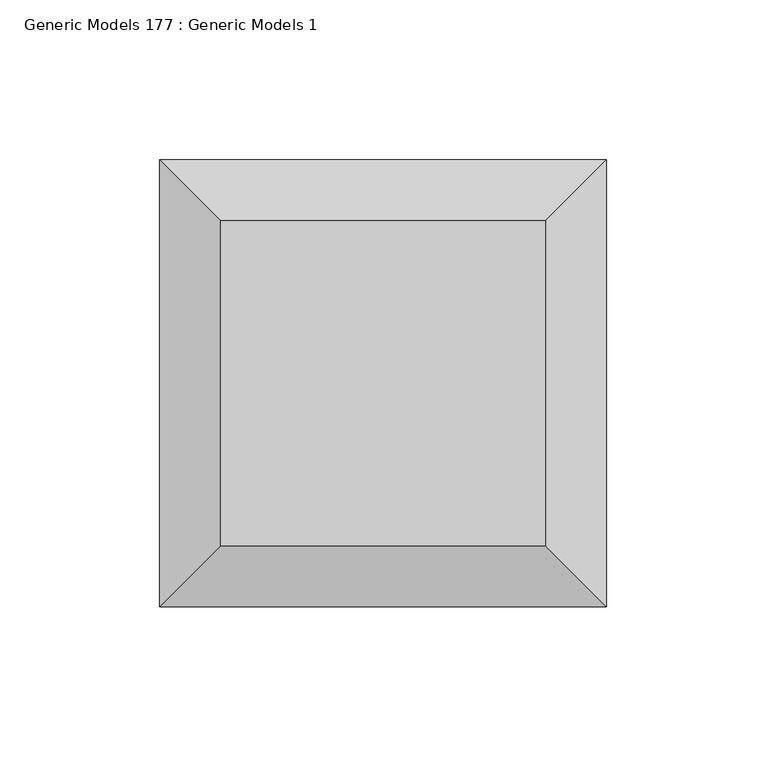
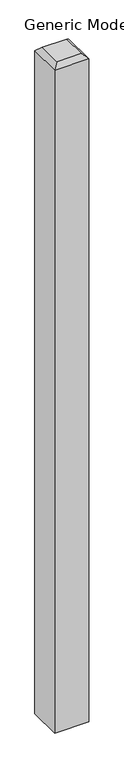
"""IFC4 building model written with IfcOpenShell, lengths in millimetres: proxy geometry, Generic Models 177 : Generic Models 1."""

from ifc_helpers import new_model, si_unit, origin, place, context, project, spatial, faceted_brep, source, transform, mapped, element, save


def generic_models_177_generic_models_1_1d143019(model_context):
    return source(origin(), model_context, "Body", "Brep", [
        faceted_brep([(56665.8125, 528.6375, -1066.8), (56526.1125, 528.6375, -1066.8), (56526.1125, 528.6375, 1809.75), (56665.8125, 528.6375, 1809.75), (56665.8125, 388.9375, -1066.8), (56665.8125, 388.9375, 1809.75), (56526.1125, 388.9375, 1809.75), (56526.1125, 388.9375, -1066.8), (56545.1625, 407.9875, 1828.8), (56646.7625, 407.9875, 1828.8), (56646.7625, 509.5875, 1828.8), (56545.1625, 509.5875, 1828.8)], [[[0, 1, 2, 3]], [[4, 5, 6, 7]], [[1, 0, 4, 7]], [[2, 1, 7, 6]], [[8, 9, 10, 11]], [[0, 3, 5, 4]], [[2, 6, 8, 11]], [[5, 3, 10, 9]], [[6, 5, 9, 8]], [[3, 2, 11, 10]]]),
    ])


if __name__ == "__main__":
    model = new_model("IFC4")
    model_context = context("Model", 3, world=origin())
    ifc_project = project(units=[si_unit("LENGTHUNIT", "METRE", prefix="MILLI")], contexts=[model_context])
    site = spatial("IfcSite", under=ifc_project)
    building = spatial("IfcBuilding", under=site)
    placement = place(None, origin())
    generic_models_177_generic_models_1_shape = generic_models_177_generic_models_1_1d143019(model_context)
    element("IfcBuildingElementProxy", 1, Name="Generic Models 177 : Generic Models 1", ObjectType="Generic Models 177 : Generic Models 1", at=placement, inside=building, context=model_context, shape_type="MappedRepresentation", body=[
        mapped(generic_models_177_generic_models_1_shape, transform((0.0, 0.0, 0.0), x_axis=(1.0, 0.0, 0.0), y_axis=(0.0, 1.0, 0.0), z_axis=(0.0, 0.0, 1.0))),
    ])
    save(model, "model.ifc")

# Revit data of these elements
# Element 1 (IfcBuildingElementProxy, "Generic Models 177 : Generic Models 1")
#   Materials on its faces: "TREATED 6X6 POST"
# Materials
#   "TREATED 6X6 POST": class "Wood", colour RGB 234 198 147, transparency 0, Description = "Pinus Echinata", Cost = 0
